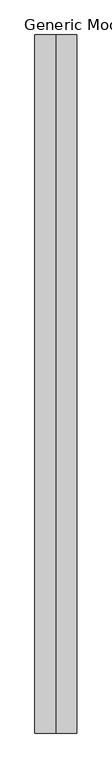
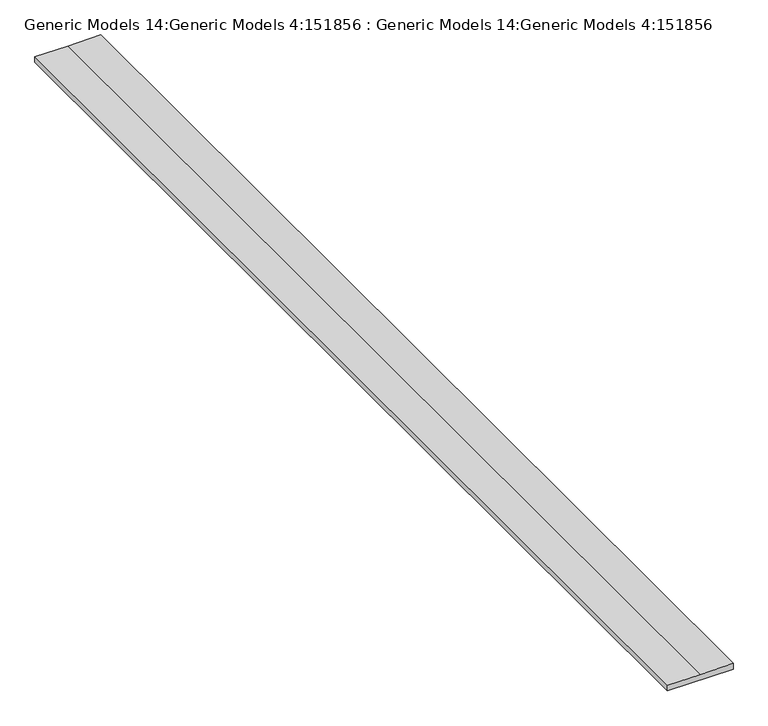
"""IFC4 building model written with IfcOpenShell, lengths in millimetres: proxy geometry, Generic Models 14:Generic Models 4:151856 : Generic Models 14:Generic Models 4:151856."""

from ifc_helpers import new_model, si_unit, frame, origin, place, context, project, spatial, polyline, outline, extrude, source, transform, mapped, element, save


def generic_models_14_generic_models_4_151856_generic_models_14_78d0f831(model_context):
    return source(origin(), model_context, "Body", "SweptSolid", [
        extrude(outline(polyline([(3590.6576609, 7235.703213), (3486.15, 7235.703213), (3486.15, 8353.303213), (3590.6576609, 8353.303213), (3579.0159942, 7794.503213), (3590.6576609, 7235.703213)])), frame((0.0, -6674.7974793, 0.0), z_axis=(0.0, 1.0, 0.0), x_axis=(0.0, 0.0, 1.0)), (0.0, 0.0, 1.0), 18643.6),
    ])


if __name__ == "__main__":
    model = new_model("IFC4")
    model_context = context("Model", 3, world=origin())
    ifc_project = project(units=[si_unit("LENGTHUNIT", "METRE", prefix="MILLI")], contexts=[model_context])
    site = spatial("IfcSite", under=ifc_project)
    building = spatial("IfcBuilding", under=site)
    placement = place(None, origin())
    generic_models_14_generic_models_4_151856_generic_models_14_shape = generic_models_14_generic_models_4_151856_generic_models_14_78d0f831(model_context)
    element("IfcBuildingElementProxy", 1, Name="Generic Models 14:Generic Models 4:151856 : Generic Models 14:Generic Models 4:151856", ObjectType="Generic Models 14:Generic Models 4:151856 : Generic Models 14:Generic Models 4:151856", at=placement, inside=building, context=model_context, shape_type="MappedRepresentation", body=[
        mapped(generic_models_14_generic_models_4_151856_generic_models_14_shape, transform((0.0, 0.0, 0.0), x_axis=(1.0, 0.0, 0.0), y_axis=(0.0, 1.0, 0.0), z_axis=(0.0, 0.0, 1.0))),
    ])
    save(model, "model.ifc")

# Revit data of these elements
# Type "Generic Models 14:Generic Models 4:151856 : Generic Models 14:Generic Models 4:151856"
#   NameOverride = "Generic Models 14:Generic Models 4:151856"
#   ObjectTypeOverride = "Generic Models 14:Generic Models 4"
#   Reference = "Generic Models 4"
#   Category = "Generic Models"
#   Tag = "151856"
# Element 1 (IfcBuildingElementProxy, "Generic Models 14:Generic Models 4:151856 : Generic Models 14:Generic Models 4:151856")
#   Materials on its faces: "_TAPERED 2X BLOCKING (1% SLOPE) - SLOPED TOWARD DRAINS (SEE ROOF PLAN) 1082"
# Materials
#   "_TAPERED 2X BLOCKING (1% SLOPE) - SLOPED TOWARD DRAINS (SEE ROOF PLAN) 1082": class "Unassigned", colour RGB 177 130 114, transparency 0
